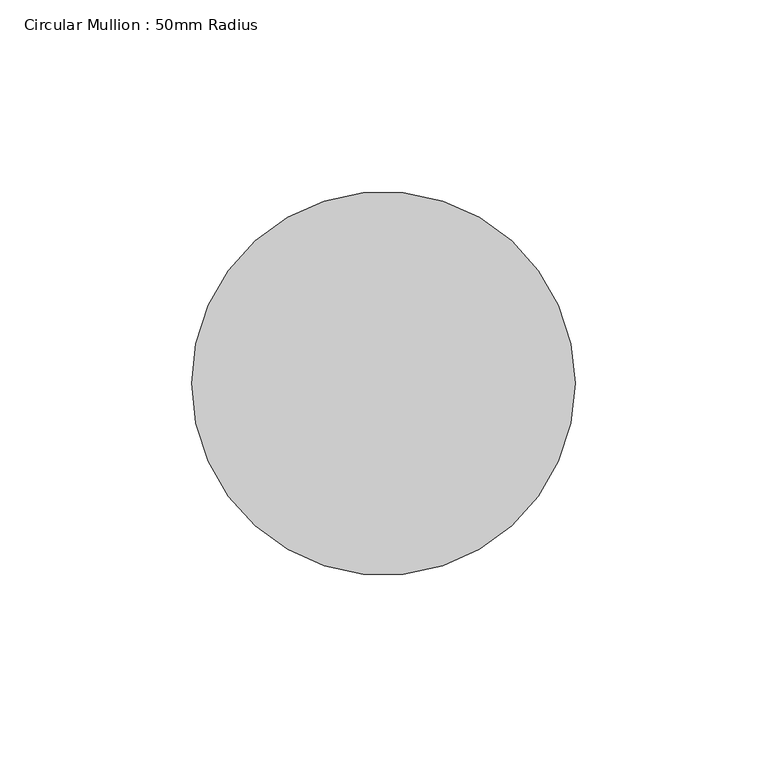
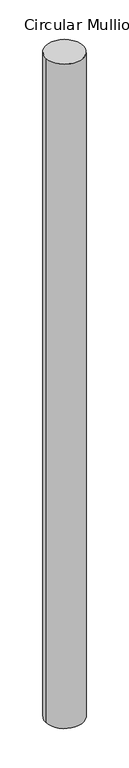
"""IFC4 building model written with IfcOpenShell, lengths in millimetres: member geometry, Circular Mullion : 50mm Radius."""

from ifc_helpers import new_model, si_unit, point, frame, origin, origin_2d, place, context, project, spatial, circle_curve, trimmed, segment, composite_curve, outline, extrude, source, transform, mapped, element, save


def circular_mullion_50mm_radius_b8d0a95c(model_context):
    return source(origin(), model_context, "Body", "SweptSolid", [
        extrude(outline(composite_curve([segment(trimmed(circle_curve(origin_2d(), 50.0), [point((50.0, 0.0))], [point((-50.0, 0.0))], False, "CARTESIAN"), True, "CONTINUOUS"), segment(trimmed(circle_curve(origin_2d(), 50.0), [point((-50.0, 0.0))], [point((50.0, 0.0))], False, "CARTESIAN"), True, "CONTINUOUS")], self_intersect=False)), frame((0.0, 0.0, -1875.1370531), z_axis=(0.0, 0.0, 1.0), x_axis=(1.0, 0.0, 0.0)), (0.0, 0.0, 1.0), 1875.1370531),
    ])


if __name__ == "__main__":
    model = new_model("IFC4")
    model_context = context("Model", 3, world=origin())
    ifc_project = project(units=[si_unit("LENGTHUNIT", "METRE", prefix="MILLI")], contexts=[model_context])
    site = spatial("IfcSite", under=ifc_project)
    building = spatial("IfcBuilding", under=site)
    placement = place(None, origin())
    circular_mullion_50mm_radius_shape = circular_mullion_50mm_radius_b8d0a95c(model_context)
    element("IfcMember", 1, ObjectType="Circular Mullion : 50mm Radius", at=placement, inside=building, context=model_context, shape_type="MappedRepresentation", body=[
        mapped(circular_mullion_50mm_radius_shape, transform((0.0, 0.0, 0.0), x_axis=(1.0, 0.0, 0.0), y_axis=(0.0, 1.0, 0.0), z_axis=(0.0, 0.0, 1.0))),
    ])
    save(model, "model.ifc")

# Revit data of these elements
# Type "Circular Mullion : 50mm Radius"
#   built-in parameter 1007350 = 0.164042 (stored number, unit not read)
# Element 1 (IfcMember, "Circular Mullion : 50mm Radius")
#   Materials on its faces: "Aluminium"
# Materials
#   "Aluminium": class "Metal", colour RGB 247 247 247, transparency 0, Description = "Aluminium 6061", Cost = 0
